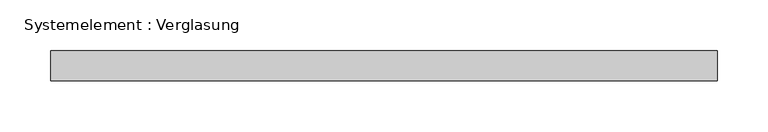
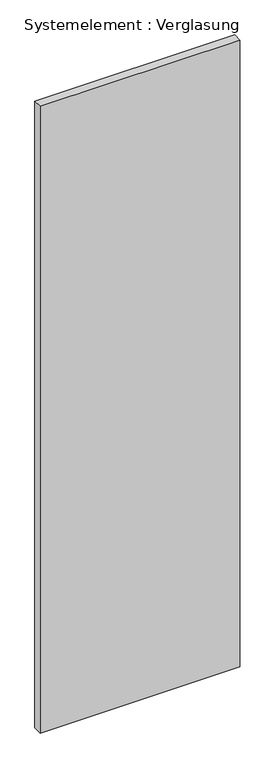
"""IFC4 building model written with IfcOpenShell, lengths in millimetres: plate geometry, Systemelement : Verglasung."""

from ifc_helpers import new_model, si_unit, origin, origin_with_axes, place, context, project, spatial, polyline, outline, extrude, source, transform, mapped, element, save


def systemelement_verglasung_ac39db88(model_context):
    return source(origin(), model_context, "Body", "SweptSolid", [
        extrude(outline(polyline([(330.143661, -15.0), (-330.143661, -15.0), (-330.143661, 15.0), (330.143661, 15.0), (330.143661, -15.0)])), origin_with_axes(), (0.0, 0.0, 1.0), 2190.0),
    ])


if __name__ == "__main__":
    model = new_model("IFC4")
    model_context = context("Model", 3, world=origin())
    ifc_project = project(units=[si_unit("LENGTHUNIT", "METRE", prefix="MILLI")], contexts=[model_context])
    site = spatial("IfcSite", under=ifc_project)
    building = spatial("IfcBuilding", under=site)
    placement = place(None, origin())
    systemelement_verglasung_shape = systemelement_verglasung_ac39db88(model_context)
    element("IfcPlate", 1, ObjectType="Systemelement : Verglasung", at=placement, inside=building, context=model_context, shape_type="MappedRepresentation", body=[
        mapped(systemelement_verglasung_shape, transform((0.0, 0.0, 0.0), x_axis=(1.0, 0.0, 0.0), y_axis=(0.0, 1.0, 0.0), z_axis=(0.0, 0.0, 1.0))),
    ])
    save(model, "model.ifc")

# Revit data of these elements
# Type "Systemelement : Verglasung"
#   Construction Type Id = "GSP4R"
#   Analytic Construction = "1/8 Zoll Pilkington-Verglasung einfach"
#   Visual Light Transmittance = 0.9
#   Solar Heat Gain Coefficient = 0.86
#   Heat Transfer Coefficient (U) = 6.7069 W/(m²·K)
# Element 1 (IfcPlate, "Systemelement : Verglasung")
#   Materials on its faces: "Glas"
# Materials
#   "Glas": class "Glas", colour RGB 0 0 255, transparency 0.75, Comments = "Render-Darstellung nicht aktualisiert ", Cost = 0
